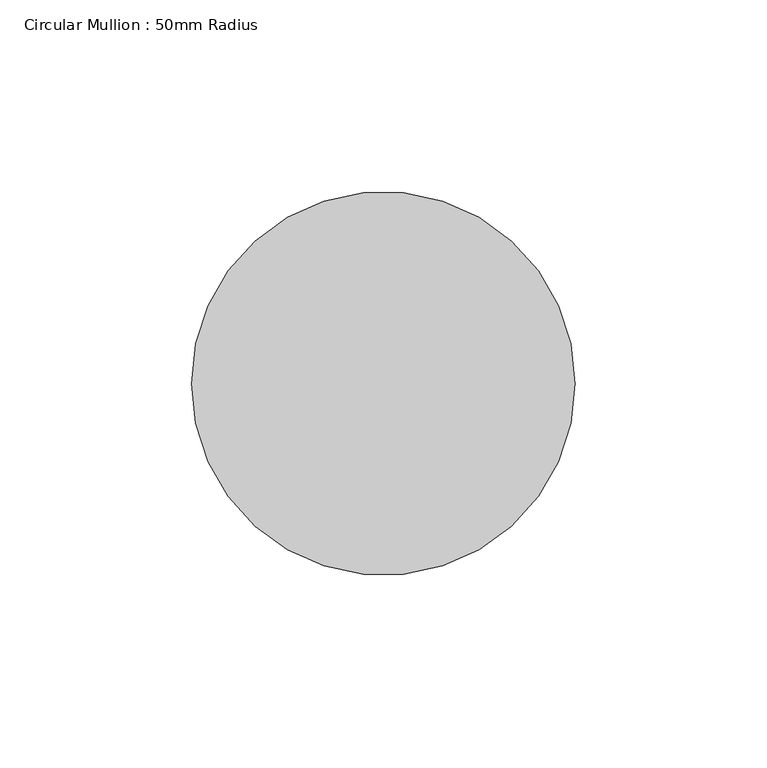
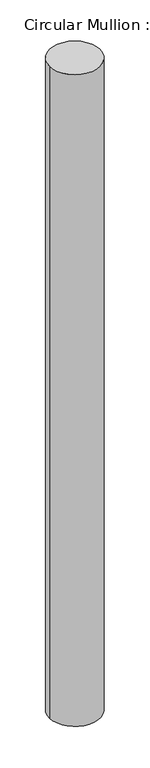
"""IFC4 building model written with IfcOpenShell, lengths in millimetres: member geometry, Circular Mullion : 50mm Radius."""

from ifc_helpers import new_model, si_unit, point, frame, origin, origin_2d, place, context, project, spatial, circle_curve, trimmed, segment, composite_curve, outline, extrude, source, transform, mapped, element, save


def circular_mullion_50mm_radius_3e261cf8(model_context):
    return source(origin(), model_context, "Body", "SweptSolid", [
        extrude(outline(composite_curve([segment(trimmed(circle_curve(origin_2d(), 50.0), [point((50.0, 0.0))], [point((-50.0, 0.0))], False, "CARTESIAN"), True, "CONTINUOUS"), segment(trimmed(circle_curve(origin_2d(), 50.0), [point((-50.0, 0.0))], [point((50.0, 0.0))], False, "CARTESIAN"), True, "CONTINUOUS")], self_intersect=False)), frame((0.0, 0.0, -1356.1740044), z_axis=(0.0, 0.0, 1.0), x_axis=(1.0, 0.0, 0.0)), (0.0, 0.0, 1.0), 1356.1740044),
    ])


if __name__ == "__main__":
    model = new_model("IFC4")
    model_context = context("Model", 3, world=origin())
    ifc_project = project(units=[si_unit("LENGTHUNIT", "METRE", prefix="MILLI")], contexts=[model_context])
    site = spatial("IfcSite", under=ifc_project)
    building = spatial("IfcBuilding", under=site)
    placement = place(None, origin())
    circular_mullion_50mm_radius_shape = circular_mullion_50mm_radius_3e261cf8(model_context)
    element("IfcMember", 1, ObjectType="Circular Mullion : 50mm Radius", at=placement, inside=building, context=model_context, shape_type="MappedRepresentation", body=[
        mapped(circular_mullion_50mm_radius_shape, transform((0.0, 0.0, 0.0), x_axis=(1.0, 0.0, 0.0), y_axis=(0.0, 1.0, 0.0), z_axis=(0.0, 0.0, 1.0))),
    ])
    save(model, "model.ifc")

# Revit data of these elements
# Type "Circular Mullion : 50mm Radius"
#   built-in parameter 1007350 = 0.164042 (stored number, unit not read)
# Element 1 (IfcMember, "Circular Mullion : 50mm Radius")
#   Materials on its faces: "Aluminium"
# Materials
#   "Aluminium": class "Metal", colour RGB 247 247 247, transparency 0, Description = "Aluminium 6061", Cost = 0
